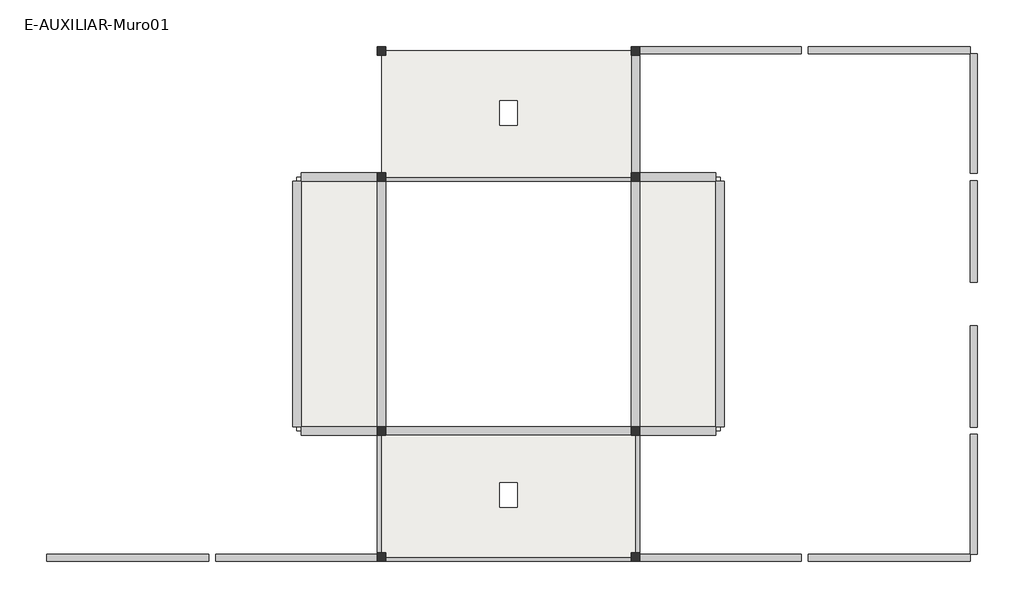
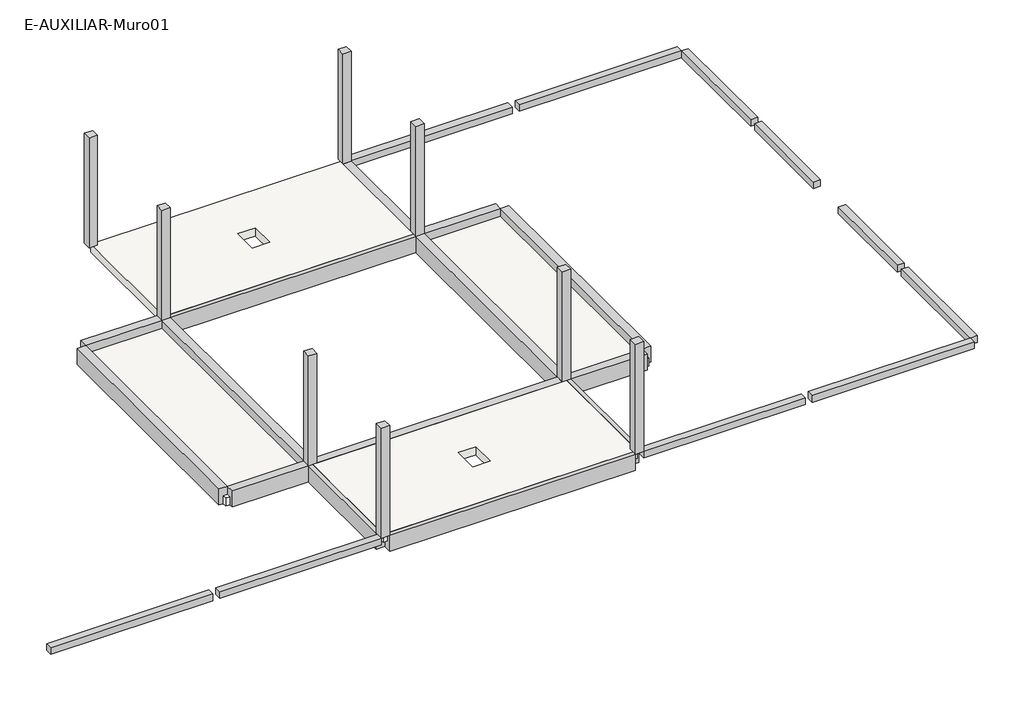
# One storey: 24 beams, 8 columns, 4 slabs.
"""IFC4 building model written with IfcOpenShell, lengths in millimetres."""

from ifc_helpers import new_model, si_unit, frame, origin, place, context, project, spatial, polyline, outline, extrude, faceted_brep, element, save

model = new_model("IFC4")

# Units and contexts
model_context = context("Model", 3, world=origin())
ifc_project = project(units=[si_unit("LENGTHUNIT", "METRE", prefix="MILLI")], contexts=[model_context])

# Site, building, storey
site = spatial("IfcSite", under=ifc_project)
building = spatial("IfcBuilding", under=site)
storey = spatial("IfcBuildingStorey", under=building, Name="E-AUXILIAR-Muro01", Elevation=2730.0)

# Beams
placement = place(None, origin())
element("IfcBeam", 1, ObjectType="E-VIGA-Hormigon : E-VIGA-Hormigon", at=placement, inside=storey, context=model_context, shape_type="Brep", body=[
    faceted_brep([(-24150.0, -13350.0, 2130.0), (-24150.0, -13350.0, 2730.0), (-24150.0, -4650.0, 2730.0), (-24150.0, -4650.0, 2130.0), (-23850.0, -13350.0, 2130.0), (-24000.0, -13350.0, 2130.0), (-24000.0, -4650.0, 2130.0), (-23850.0, -4650.0, 2130.0), (-23850.0, -13350.0, 2730.0), (-23850.0, -13350.0, 2430.0), (-23850.0, -4650.0, 2430.0), (-23850.0, -4650.0, 2730.0)], [[[0, 1, 2, 3]], [[4, 5, 0, 3, 6, 7]], [[8, 9, 4, 7, 10, 11]], [[1, 8, 11, 2]], [[2, 11, 10, 7, 6, 3]], [[1, 0, 5, 4, 9, 8]]]),
])
element("IfcBeam", 2, ObjectType="E-VIGA-Hormigon : E-VIGA-Hormigon", at=placement, inside=storey, context=model_context, shape_type="Brep", body=[
    faceted_brep([(-21150.0, -13350.0, 2130.0), (-21150.0, -13350.0, 2430.0), (-21150.0, -13350.0, 2730.0), (-21150.0, -4650.0, 2730.0), (-21150.0, -4650.0, 2430.0), (-21150.0, -4650.0, 2130.0), (-20850.0, -13350.0, 2130.0), (-21000.0, -13350.0, 2130.0), (-21000.0, -4650.0, 2130.0), (-20850.0, -4650.0, 2130.0), (-20850.0, -13350.0, 2730.0), (-20850.0, -4650.0, 2730.0)], [[[0, 1, 2, 3, 4, 5]], [[6, 7, 0, 5, 8, 9]], [[10, 6, 9, 11]], [[2, 10, 11, 3]], [[3, 11, 9, 8, 5, 4]], [[2, 1, 0, 7, 6, 10]]]),
])
element("IfcBeam", 3, ObjectType="E-VIGA-Hormigon : E-VIGA-Hormigon", at=placement, inside=storey, context=model_context, shape_type="Brep", body=[
    faceted_brep([(-12150.0, -13350.0, 2130.0), (-12150.0, -13350.0, 2730.0), (-12150.0, -4650.0, 2730.0), (-12150.0, -4650.0, 2130.0), (-11850.0, -13350.0, 2130.0), (-12000.0, -13350.0, 2130.0), (-12000.0, -4650.0, 2130.0), (-11850.0, -4650.0, 2130.0), (-11850.0, -13350.0, 2730.0), (-11850.0, -13350.0, 2430.0), (-11850.0, -4650.0, 2430.0), (-11850.0, -4650.0, 2730.0)], [[[0, 1, 2, 3]], [[4, 5, 0, 3, 6, 7]], [[8, 9, 4, 7, 10, 11]], [[1, 8, 11, 2]], [[2, 11, 10, 7, 6, 3]], [[1, 0, 5, 4, 9, 8]]]),
])
element("IfcBeam", 4, ObjectType="E-VIGA-Hormigon : E-VIGA-Hormigon", at=placement, inside=storey, context=model_context, shape_type="Brep", body=[
    faceted_brep([(-9150.0, -13350.0, 2130.0), (-9150.0, -13350.0, 2430.0), (-9150.0, -13350.0, 2730.0), (-9150.0, -4650.0, 2730.0), (-9150.0, -4650.0, 2430.0), (-9150.0, -4650.0, 2130.0), (-8850.0, -13350.0, 2130.0), (-9000.0, -13350.0, 2130.0), (-9000.0, -4650.0, 2130.0), (-8850.0, -4650.0, 2130.0), (-8850.0, -13350.0, 2730.0), (-8850.0, -4650.0, 2730.0)], [[[0, 1, 2, 3, 4, 5]], [[6, 7, 0, 5, 8, 9]], [[10, 6, 9, 11]], [[2, 10, 11, 3]], [[3, 11, 9, 8, 5, 4]], [[2, 1, 0, 7, 6, 10]]]),
])
element("IfcBeam", 5, ObjectType="E-VIGA-Hormigon : E-VIGA-Hormigon", at=placement, inside=storey, context=model_context, shape_type="SweptSolid", body=[
    extrude(outline(polyline([(-4650.0, 2730.0), (-4350.0, 2730.0), (-4350.0, 2130.0), (-4500.0, 2130.0), (-4500.0, 2430.0), (-4650.0, 2430.0), (-4650.0, 2730.0)])), frame((-23850.0, 0.0, 0.0), z_axis=(1.0, 0.0, 0.0), x_axis=(0.0, 1.0, 0.0)), (0.0, 0.0, 1.0), 2700.0),
])
element("IfcBeam", 6, ObjectType="E-VIGA-Hormigon : E-VIGA-Hormigon", at=placement, inside=storey, context=model_context, shape_type="SweptSolid", body=[
    extrude(outline(polyline([(-4350.0, 2130.0), (-4650.0, 2130.0), (-4650.0, 2730.0), (-4500.0, 2730.0), (-4500.0, 2430.0), (-4350.0, 2430.0), (-4350.0, 2130.0)])), frame((-20850.0, 0.0, 0.0), z_axis=(1.0, 0.0, 0.0), x_axis=(0.0, 1.0, 0.0)), (0.0, 0.0, 1.0), 8700.0),
])
element("IfcBeam", 7, ObjectType="E-VIGA-Hormigon : E-VIGA-Hormigon", at=placement, inside=storey, context=model_context, shape_type="SweptSolid", body=[
    extrude(outline(polyline([(-4650.0, 2730.0), (-4350.0, 2730.0), (-4350.0, 2130.0), (-4500.0, 2130.0), (-4500.0, 2430.0), (-4650.0, 2430.0), (-4650.0, 2730.0)])), frame((-11850.0, 0.0, 0.0), z_axis=(1.0, 0.0, 0.0), x_axis=(0.0, 1.0, 0.0)), (0.0, 0.0, 1.0), 2700.0),
])
element("IfcBeam", 8, ObjectType="E-VIGA-Hormigon : E-VIGA-Hormigon", at=placement, inside=storey, context=model_context, shape_type="SweptSolid", body=[
    extrude(outline(polyline([(-13650.0, 2130.0), (-13650.0, 2730.0), (-13350.0, 2730.0), (-13350.0, 2430.0), (-13500.0, 2430.0), (-13500.0, 2130.0), (-13650.0, 2130.0)])), frame((-23850.0, 0.0, 0.0), z_axis=(1.0, 0.0, 0.0), x_axis=(0.0, 1.0, 0.0)), (0.0, 0.0, 1.0), 2700.0),
])
element("IfcBeam", 9, ObjectType="E-VIGA-Hormigon : E-VIGA-Hormigon", at=placement, inside=storey, context=model_context, shape_type="Brep", body=[
    faceted_brep([(-12150.0, -13350.0, 2130.0), (-20850.0, -13350.0, 2130.0), (-20850.0, -13350.0, 2730.0), (-12150.0, -13350.0, 2730.0), (-12150.0, -13650.0, 2130.0), (-20850.0, -13650.0, 2130.0), (-12150.0, -13650.0, 2730.0), (-20850.0, -13650.0, 2730.0), (-20850.0, -13650.0, 2430.0), (-12150.0, -13650.0, 2430.0), (-20850.0, -13500.0, 2730.0), (-12150.0, -13500.0, 2730.0)], [[[0, 1, 2, 3]], [[4, 5, 1, 0]], [[6, 7, 8, 5, 4, 9]], [[3, 2, 10, 7, 6, 11]], [[3, 11, 6, 9, 4, 0]], [[2, 1, 5, 8, 7, 10]]]),
])
element("IfcBeam", 10, ObjectType="E-VIGA-Hormigon : E-VIGA-Hormigon", at=placement, inside=storey, context=model_context, shape_type="SweptSolid", body=[
    extrude(outline(polyline([(-13650.0, 2130.0), (-13650.0, 2730.0), (-13350.0, 2730.0), (-13350.0, 2430.0), (-13500.0, 2430.0), (-13500.0, 2130.0), (-13650.0, 2130.0)])), frame((-11850.0, 0.0, 0.0), z_axis=(1.0, 0.0, 0.0), x_axis=(0.0, 1.0, 0.0)), (0.0, 0.0, 1.0), 2700.0),
])
element("IfcBeam", 11, ObjectType="E-VIGA-Hormigon : E-VIGA-Hormigon", at=placement, inside=storey, context=model_context, shape_type="SweptSolid", body=[
    extrude(outline(polyline([(2730.0, -21150.0), (2130.0, -21150.0), (2130.0, -20850.0), (2430.0, -20850.0), (2430.0, -21000.0), (2730.0, -21000.0), (2730.0, -21150.0)])), frame((0.0, -17825.0, 0.0), z_axis=(0.0, 1.0, 0.0), x_axis=(0.0, 0.0, 1.0)), (0.0, 0.0, 1.0), 4175.0),
])
element("IfcBeam", 12, ObjectType="E-VIGA-Hormigon : E-VIGA-Hormigon", at=placement, inside=storey, context=model_context, shape_type="Brep", body=[
    faceted_brep([(-11850.0, -4350.0, 2130.0), (-11850.0, -175.0, 2130.0), (-11850.0, -175.0, 2730.0), (-11850.0, -4350.0, 2730.0), (-12150.0, -4350.0, 2130.0), (-12150.0, -175.0, 2130.0), (-12150.0, -4350.0, 2730.0), (-12150.0, -175.0, 2730.0), (-12150.0, -175.0, 2430.0), (-12150.0, -4350.0, 2430.0), (-12000.0, -175.0, 2730.0), (-12000.0, -4350.0, 2730.0)], [[[0, 1, 2, 3]], [[4, 5, 1, 0]], [[6, 7, 8, 5, 4, 9]], [[3, 2, 10, 7, 6, 11]], [[3, 11, 6, 9, 4, 0]], [[2, 1, 5, 8, 7, 10]]]),
])
element("IfcBeam", 13, ObjectType="E-VIGA-Hormigon : E-VIGA-Hormigon", at=placement, inside=storey, context=model_context, shape_type="SweptSolid", body=[
    extrude(outline(polyline([(2130.0, -12150.0), (2130.0, -11850.0), (2730.0, -11850.0), (2730.0, -12000.0), (2430.0, -12000.0), (2430.0, -12150.0), (2130.0, -12150.0)])), frame((0.0, -17825.0, 0.0), z_axis=(0.0, 1.0, 0.0), x_axis=(0.0, 0.0, 1.0)), (0.0, 0.0, 1.0), 4175.0),
])
element("IfcBeam", 14, ObjectType="E-VIGA-Hormigon : E-VIGA-Hormigon", at=placement, inside=storey, context=model_context, shape_type="SweptSolid", body=[
    extrude(outline(polyline([(-17825.0, 2130.0), (-18125.0, 2130.0), (-18125.0, 2730.0), (-17975.0, 2730.0), (-17975.0, 2430.0), (-17825.0, 2430.0), (-17825.0, 2130.0)])), frame((-20850.0, 0.0, 0.0), z_axis=(1.0, 0.0, 0.0), x_axis=(0.0, 1.0, 0.0)), (0.0, 0.0, 1.0), 8700.0),
])
element("IfcBeam", 15, ObjectType="E-VIGA-Hormigon : E-VIGA-Hormigon", at=placement, inside=storey, context=model_context, shape_type="SweptSolid", body=[
    extrude(outline(polyline([(-125.0, -13625.0), (125.0, -13625.0), (125.0, -17875.0), (-125.0, -17875.0), (-125.0, -13625.0)])), frame((0.0, 0.0, 2480.0), z_axis=(0.0, 0.0, 1.0), x_axis=(1.0, 0.0, 0.0)), (0.0, 0.0, 1.0), 250.0),
])
element("IfcBeam", 16, ObjectType="E-VIGA-Hormigon : E-VIGA-Hormigon", at=placement, inside=storey, context=model_context, shape_type="SweptSolid", body=[
    extrude(outline(polyline([(125.0, -13375.0), (-125.0, -13375.0), (-125.0, -9775.0), (125.0, -9775.0), (125.0, -13375.0)])), frame((0.0, 0.0, 2480.0), z_axis=(0.0, 0.0, 1.0), x_axis=(1.0, 0.0, 0.0)), (0.0, 0.0, 1.0), 250.0),
])
element("IfcBeam", 17, ObjectType="E-VIGA-Hormigon : E-VIGA-Hormigon", at=placement, inside=storey, context=model_context, shape_type="SweptSolid", body=[
    extrude(outline(polyline([(-125.0, -4625.0), (125.0, -4625.0), (125.0, -8225.0), (-125.0, -8225.0), (-125.0, -4625.0)])), frame((0.0, 0.0, 2480.0), z_axis=(0.0, 0.0, 1.0), x_axis=(1.0, 0.0, 0.0)), (0.0, 0.0, 1.0), 250.0),
])
element("IfcBeam", 18, ObjectType="E-VIGA-Hormigon : E-VIGA-Hormigon", at=placement, inside=storey, context=model_context, shape_type="SweptSolid", body=[
    extrude(outline(polyline([(125.0, -125.0), (125.0, -4375.0), (-125.0, -4375.0), (-125.0, -125.0), (125.0, -125.0)])), frame((0.0, 0.0, 2480.0), z_axis=(0.0, 0.0, 1.0), x_axis=(1.0, 0.0, 0.0)), (0.0, 0.0, 1.0), 250.0),
])
element("IfcBeam", 19, ObjectType="E-VIGA-Hormigon : E-VIGA-Hormigon", at=placement, inside=storey, context=model_context, shape_type="SweptSolid", body=[
    extrude(outline(polyline([(-5875.0, 125.0), (-125.0, 125.0), (-125.0, -125.0), (-5875.0, -125.0), (-5875.0, 125.0)])), frame((0.0, 0.0, 2480.0), z_axis=(0.0, 0.0, 1.0), x_axis=(1.0, 0.0, 0.0)), (0.0, 0.0, 1.0), 250.0),
])
element("IfcBeam", 20, ObjectType="E-VIGA-Hormigon : E-VIGA-Hormigon", at=placement, inside=storey, context=model_context, shape_type="SweptSolid", body=[
    extrude(outline(polyline([(-6125.0, 125.0), (-6125.0, -125.0), (-11850.0, -125.0), (-11850.0, 125.0), (-6125.0, 125.0)])), frame((0.0, 0.0, 2480.0), z_axis=(0.0, 0.0, 1.0), x_axis=(1.0, 0.0, 0.0)), (0.0, 0.0, 1.0), 250.0),
])
element("IfcBeam", 21, ObjectType="E-VIGA-Hormigon : E-VIGA-Hormigon", at=placement, inside=storey, context=model_context, shape_type="SweptSolid", body=[
    extrude(outline(polyline([(-27125.0, -18125.0), (-32875.0, -18125.0), (-32875.0, -17875.0), (-27125.0, -17875.0), (-27125.0, -18125.0)])), frame((0.0, 0.0, 2480.0), z_axis=(0.0, 0.0, 1.0), x_axis=(1.0, 0.0, 0.0)), (0.0, 0.0, 1.0), 250.0),
])
element("IfcBeam", 22, ObjectType="E-VIGA-Hormigon : E-VIGA-Hormigon", at=placement, inside=storey, context=model_context, shape_type="SweptSolid", body=[
    extrude(outline(polyline([(-26875.0, -18125.0), (-26875.0, -17875.0), (-21150.0, -17875.0), (-21150.0, -18125.0), (-26875.0, -18125.0)])), frame((0.0, 0.0, 2480.0), z_axis=(0.0, 0.0, 1.0), x_axis=(1.0, 0.0, 0.0)), (0.0, 0.0, 1.0), 250.0),
])
element("IfcBeam", 23, ObjectType="E-VIGA-Hormigon : E-VIGA-Hormigon", at=placement, inside=storey, context=model_context, shape_type="SweptSolid", body=[
    extrude(outline(polyline([(-5875.0, -18125.0), (-5875.0, -17875.0), (-125.0, -17875.0), (-125.0, -18125.0), (-5875.0, -18125.0)])), frame((0.0, 0.0, 2480.0), z_axis=(0.0, 0.0, 1.0), x_axis=(1.0, 0.0, 0.0)), (0.0, 0.0, 1.0), 250.0),
])
element("IfcBeam", 24, ObjectType="E-VIGA-Hormigon : E-VIGA-Hormigon", at=placement, inside=storey, context=model_context, shape_type="SweptSolid", body=[
    extrude(outline(polyline([(-6125.0, -17875.0), (-6125.0, -18125.0), (-11850.0, -18125.0), (-11850.0, -17875.0), (-6125.0, -17875.0)])), frame((0.0, 0.0, 2480.0), z_axis=(0.0, 0.0, 1.0), x_axis=(1.0, 0.0, 0.0)), (0.0, 0.0, 1.0), 250.0),
])

# Columns
element("IfcColumn", 25, ObjectType="Hormigón-Cuadrado-Pilar : PILAR 30X30", at=placement, inside=storey, context=model_context, shape_type="SweptSolid", body=[
    extrude(outline(polyline([(-20850.0, -4350.0), (-20850.0, -4650.0), (-21150.0, -4650.0), (-21150.0, -4350.0), (-20850.0, -4350.0)])), frame((0.0, 0.0, 2730.0), z_axis=(0.0, 0.0, 1.0), x_axis=(1.0, 0.0, 0.0)), (0.0, 0.0, 1.0), 4120.0),
])
element("IfcColumn", 26, ObjectType="Hormigón-Cuadrado-Pilar : PILAR 30X30", at=placement, inside=storey, context=model_context, shape_type="Brep", body=[
    faceted_brep([(-11850.0, -4350.0, 2730.0), (-11850.0, -4650.0, 2730.0), (-12150.0, -4650.0, 2730.0), (-12150.0, -4350.0, 2730.0), (-12000.0, -4350.0, 2730.0), (-11850.0, -4350.0, 6850.0), (-11850.0, -4650.0, 6850.0), (-12150.0, -4650.0, 6850.0), (-12150.0, -4350.0, 6850.0)], [[[0, 1, 2, 3, 4]], [[5, 6, 1, 0]], [[6, 7, 2, 1]], [[7, 8, 3, 2]], [[8, 5, 0, 4, 3]], [[5, 8, 7, 6]]]),
])
element("IfcColumn", 27, ObjectType="Hormigón-Cuadrado-Pilar : PILAR 30X30", at=placement, inside=storey, context=model_context, shape_type="Brep", body=[
    faceted_brep([(-11850.0, -13350.0, 2730.0), (-11850.0, -13650.0, 2730.0), (-12150.0, -13650.0, 2730.0), (-12150.0, -13500.0, 2730.0), (-12150.0, -13350.0, 2730.0), (-11850.0, -13350.0, 6850.0), (-11850.0, -13650.0, 6850.0), (-12150.0, -13650.0, 6850.0), (-12150.0, -13350.0, 6850.0)], [[[0, 1, 2, 3, 4]], [[5, 6, 1, 0]], [[6, 7, 2, 1]], [[7, 8, 4, 3, 2]], [[8, 5, 0, 4]], [[5, 8, 7, 6]]]),
])
element("IfcColumn", 28, ObjectType="Hormigón-Cuadrado-Pilar : PILAR 30X30", at=placement, inside=storey, context=model_context, shape_type="Brep", body=[
    faceted_brep([(-20850.0, -13350.0, 2730.0), (-20850.0, -13500.0, 2730.0), (-20850.0, -13650.0, 2730.0), (-21150.0, -13650.0, 2730.0), (-21150.0, -13350.0, 2730.0), (-20850.0, -13350.0, 6850.0), (-20850.0, -13650.0, 6850.0), (-21150.0, -13650.0, 6850.0), (-21150.0, -13350.0, 6850.0)], [[[0, 1, 2, 3, 4]], [[5, 6, 2, 1, 0]], [[6, 7, 3, 2]], [[7, 8, 4, 3]], [[8, 5, 0, 4]], [[5, 8, 7, 6]]]),
])
element("IfcColumn", 29, ObjectType="Hormigón-Cuadrado-Pilar : PILAR 30X30", at=placement, inside=storey, context=model_context, shape_type="SweptSolid", body=[
    extrude(outline(polyline([(-20850.0, -17825.0), (-20850.0, -18125.0), (-21150.0, -18125.0), (-21150.0, -17825.0), (-20850.0, -17825.0)])), frame((0.0, 0.0, 2730.0), z_axis=(0.0, 0.0, 1.0), x_axis=(1.0, 0.0, 0.0)), (0.0, 0.0, 1.0), 4120.0),
])
element("IfcColumn", 30, ObjectType="Hormigón-Cuadrado-Pilar : PILAR 30X30", at=placement, inside=storey, context=model_context, shape_type="SweptSolid", body=[
    extrude(outline(polyline([(-12150.0, -17825.0), (-11850.0, -17825.0), (-11850.0, -18125.0), (-12150.0, -18125.0), (-12150.0, -17825.0)])), frame((0.0, 0.0, 2730.0), z_axis=(0.0, 0.0, 1.0), x_axis=(1.0, 0.0, 0.0)), (0.0, 0.0, 1.0), 4120.0),
])
element("IfcColumn", 31, ObjectType="Hormigón-Cuadrado-Pilar : PILAR 30X30", at=placement, inside=storey, context=model_context, shape_type="SweptSolid", body=[
    extrude(outline(polyline([(-20850.0, -175.0), (-21150.0, -175.0), (-21150.0, 125.0), (-20850.0, 125.0), (-20850.0, -175.0)])), frame((0.0, 0.0, 2730.0), z_axis=(0.0, 0.0, 1.0), x_axis=(1.0, 0.0, 0.0)), (0.0, 0.0, 1.0), 4120.0),
])
element("IfcColumn", 32, ObjectType="Hormigón-Cuadrado-Pilar : PILAR 30X30", at=placement, inside=storey, context=model_context, shape_type="Brep", body=[
    faceted_brep([(-12150.0, -175.0, 2730.0), (-12150.0, 125.0, 2730.0), (-11850.0, 125.0, 2730.0), (-11850.0, -175.0, 2730.0), (-12000.0, -175.0, 2730.0), (-12150.0, -175.0, 6850.0), (-12150.0, 125.0, 6850.0), (-11850.0, 125.0, 6850.0), (-11850.0, -175.0, 6850.0)], [[[0, 1, 2, 3, 4]], [[5, 6, 1, 0]], [[6, 7, 2, 1]], [[7, 8, 3, 2]], [[8, 5, 0, 4, 3]], [[5, 8, 7, 6]]]),
])

# Slabs
element("IfcSlab", 33, ObjectType="FORJADO 1_PABLO", at=placement, inside=storey, context=model_context, shape_type="Brep", body=[
    faceted_brep([(-21000.0, -4500.0, 2430.0), (-21000.0, -4350.0, 2430.0), (-21000.0, -175.0, 2430.0), (-21000.0, -25.0, 2430.0), (-20850.0, -25.0, 2430.0), (-12150.0, -25.0, 2430.0), (-12000.0, -25.0, 2430.0), (-12000.0, -175.0, 2430.0), (-12150.0, -175.0, 2430.0), (-12150.0, -4350.0, 2430.0), (-12000.0, -4350.0, 2430.0), (-12000.0, -4500.0, 2430.0), (-12150.0, -4500.0, 2430.0), (-20850.0, -4500.0, 2430.0), (-16811.05, -1791.95, 2430.0), (-16811.05, -2668.05, 2430.0), (-16188.95, -2668.05, 2430.0), (-16188.95, -1791.95, 2430.0), (-21000.0, -25.0, 2730.0), (-21000.0, -175.0, 2730.0), (-21000.0, -4350.0, 2730.0), (-21000.0, -4500.0, 2730.0), (-20850.0, -4500.0, 2730.0), (-12150.0, -4500.0, 2730.0), (-12000.0, -4500.0, 2730.0), (-12000.0, -4350.0, 2730.0), (-12150.0, -4350.0, 2730.0), (-12150.0, -175.0, 2730.0), (-12000.0, -175.0, 2730.0), (-12000.0, -25.0, 2730.0), (-12150.0, -25.0, 2730.0), (-20850.0, -25.0, 2730.0), (-16811.05, -2668.05, 2730.0), (-16811.05, -1791.95, 2730.0), (-16188.95, -1791.95, 2730.0), (-16188.95, -2668.05, 2730.0)], [[[0, 1, 2, 3, 4, 5, 6, 7, 8, 9, 10, 11, 12, 13], [14, 15, 16, 17]], [[18, 19, 20, 21, 22, 23, 24, 25, 26, 27, 28, 29, 30, 31], [32, 33, 34, 35]], [[3, 2, 1, 0, 21, 20, 19, 18]], [[6, 5, 4, 3, 18, 31, 30, 29]], [[24, 11, 10, 25]], [[6, 29, 28, 7]], [[0, 13, 12, 11, 24, 23, 22, 21]], [[15, 14, 33, 32]], [[16, 15, 32, 35]], [[17, 16, 35, 34]], [[14, 17, 34, 33]], [[26, 9, 8, 27]], [[9, 26, 25, 10]], [[27, 8, 7, 28]]]),
])
element("IfcSlab", 34, ObjectType="FORJADO 1_PABLO", at=placement, inside=storey, context=model_context, shape_type="Brep", body=[
    faceted_brep([(-12000.0, -13500.0, 2430.0), (-12000.0, -13650.0, 2430.0), (-12000.0, -17825.0, 2430.0), (-12000.0, -17975.0, 2430.0), (-12150.0, -17975.0, 2430.0), (-20850.0, -17975.0, 2430.0), (-21000.0, -17975.0, 2430.0), (-21000.0, -17825.0, 2430.0), (-21000.0, -13650.0, 2430.0), (-21000.0, -13500.0, 2430.0), (-20850.0, -13500.0, 2430.0), (-20850.0, -13650.0, 2430.0), (-12150.0, -13650.0, 2430.0), (-12150.0, -13500.0, 2430.0), (-16188.95, -15331.95, 2430.0), (-16811.05, -15331.95, 2430.0), (-16811.05, -16208.05, 2430.0), (-16188.95, -16208.05, 2430.0), (-12000.0, -17975.0, 2730.0), (-12000.0, -17825.0, 2730.0), (-12000.0, -13650.0, 2730.0), (-12000.0, -13500.0, 2730.0), (-12150.0, -13500.0, 2730.0), (-12150.0, -13650.0, 2730.0), (-20850.0, -13650.0, 2730.0), (-20850.0, -13500.0, 2730.0), (-21000.0, -13500.0, 2730.0), (-21000.0, -13650.0, 2730.0), (-21000.0, -17825.0, 2730.0), (-21000.0, -17975.0, 2730.0), (-20850.0, -17975.0, 2730.0), (-12150.0, -17975.0, 2730.0), (-16811.05, -15331.95, 2730.0), (-16188.95, -15331.95, 2730.0), (-16188.95, -16208.05, 2730.0), (-16811.05, -16208.05, 2730.0)], [[[0, 1, 2, 3, 4, 5, 6, 7, 8, 9, 10, 11, 12, 13], [14, 15, 16, 17]], [[18, 19, 20, 21, 22, 23, 24, 25, 26, 27, 28, 29, 30, 31], [32, 33, 34, 35]], [[3, 2, 1, 0, 21, 20, 19, 18]], [[6, 5, 4, 3, 18, 31, 30, 29]], [[9, 8, 7, 6, 29, 28, 27, 26]], [[21, 0, 13, 22]], [[9, 26, 25, 10]], [[15, 14, 33, 32]], [[16, 15, 32, 35]], [[17, 16, 35, 34]], [[14, 17, 34, 33]], [[23, 12, 11, 24]], [[12, 23, 22, 13]], [[24, 11, 10, 25]]]),
])
element("IfcSlab", 35, ObjectType="FORJADO 1_PABLO", at=placement, inside=storey, context=model_context, shape_type="Brep", body=[
    faceted_brep([(-9000.0, -13500.0, 2130.0), (-9150.0, -13500.0, 2130.0), (-11850.0, -13500.0, 2130.0), (-12000.0, -13500.0, 2130.0), (-12000.0, -13350.0, 2130.0), (-11850.0, -13350.0, 2130.0), (-11850.0, -4650.0, 2130.0), (-12000.0, -4650.0, 2130.0), (-12000.0, -4500.0, 2130.0), (-11850.0, -4500.0, 2130.0), (-9150.0, -4500.0, 2130.0), (-9000.0, -4500.0, 2130.0), (-9000.0, -4650.0, 2130.0), (-9150.0, -4650.0, 2130.0), (-9150.0, -13350.0, 2130.0), (-9000.0, -13350.0, 2130.0), (-12000.0, -13500.0, 2430.0), (-11850.0, -13500.0, 2430.0), (-9150.0, -13500.0, 2430.0), (-9000.0, -13500.0, 2430.0), (-9000.0, -13350.0, 2430.0), (-9150.0, -13350.0, 2430.0), (-9150.0, -4650.0, 2430.0), (-9000.0, -4650.0, 2430.0), (-9000.0, -4500.0, 2430.0), (-9150.0, -4500.0, 2430.0), (-11850.0, -4500.0, 2430.0), (-12000.0, -4500.0, 2430.0), (-12000.0, -4650.0, 2430.0), (-11850.0, -4650.0, 2430.0), (-11850.0, -13350.0, 2430.0), (-12000.0, -13350.0, 2430.0)], [[[0, 1, 2, 3, 4, 5, 6, 7, 8, 9, 10, 11, 12, 13, 14, 15]], [[16, 17, 18, 19, 20, 21, 22, 23, 24, 25, 26, 27, 28, 29, 30, 31]], [[11, 24, 23, 12]], [[19, 0, 15, 20]], [[3, 2, 1, 0, 19, 18, 17, 16]], [[27, 8, 7, 28]], [[3, 16, 31, 4]], [[11, 10, 9, 8, 27, 26, 25, 24]], [[29, 6, 5, 30]], [[6, 29, 28, 7]], [[30, 5, 4, 31]], [[13, 22, 21, 14]], [[22, 13, 12, 23]], [[14, 21, 20, 15]]]),
])
element("IfcSlab", 36, ObjectType="FORJADO 1_PABLO", at=placement, inside=storey, context=model_context, shape_type="Brep", body=[
    faceted_brep([(-21000.0, -13500.0, 2130.0), (-21150.0, -13500.0, 2130.0), (-23850.0, -13500.0, 2130.0), (-24000.0, -13500.0, 2130.0), (-24000.0, -13350.0, 2130.0), (-23850.0, -13350.0, 2130.0), (-23850.0, -4650.0, 2130.0), (-24000.0, -4650.0, 2130.0), (-24000.0, -4500.0, 2130.0), (-23850.0, -4500.0, 2130.0), (-21150.0, -4500.0, 2130.0), (-21000.0, -4500.0, 2130.0), (-21000.0, -4650.0, 2130.0), (-21150.0, -4650.0, 2130.0), (-21150.0, -13350.0, 2130.0), (-21000.0, -13350.0, 2130.0), (-24000.0, -13500.0, 2430.0), (-23850.0, -13500.0, 2430.0), (-21150.0, -13500.0, 2430.0), (-21000.0, -13500.0, 2430.0), (-21000.0, -13350.0, 2430.0), (-21150.0, -13350.0, 2430.0), (-21150.0, -4650.0, 2430.0), (-21000.0, -4650.0, 2430.0), (-21000.0, -4500.0, 2430.0), (-21150.0, -4500.0, 2430.0), (-23850.0, -4500.0, 2430.0), (-24000.0, -4500.0, 2430.0), (-24000.0, -4650.0, 2430.0), (-23850.0, -4650.0, 2430.0), (-23850.0, -13350.0, 2430.0), (-24000.0, -13350.0, 2430.0)], [[[0, 1, 2, 3, 4, 5, 6, 7, 8, 9, 10, 11, 12, 13, 14, 15]], [[16, 17, 18, 19, 20, 21, 22, 23, 24, 25, 26, 27, 28, 29, 30, 31]], [[11, 24, 23, 12]], [[19, 0, 15, 20]], [[3, 2, 1, 0, 19, 18, 17, 16]], [[27, 8, 7, 28]], [[3, 16, 31, 4]], [[11, 10, 9, 8, 27, 26, 25, 24]], [[29, 6, 5, 30]], [[6, 29, 28, 7]], [[30, 5, 4, 31]], [[13, 22, 21, 14]], [[22, 13, 12, 23]], [[14, 21, 20, 15]]]),
])

save(model, "model.ifc")

# Revit data of these elements
# Type "E-VIGA-Hormigon : E-VIGA-Hormigon"
#   Numeration [instance default] = ""
#   Length [instance default] = 3.000 m
#   AnchoViga [instance default] = 0.200 m
#   AltoViga [instance default] = 0.300 m
# Type "Hormigón-Cuadrado-Pilar : PILAR 30X30"
#   b = 0.300 m
#   Structural Material [instance default] = Hormigón - Hormigón moldeado in situ
# Type "FORJADO 1_PABLO"
#   Function = 0
#   Layers, outside or top first: 0.140 m "Hormigón, moldeado in situ" (function 1); 0.160 m "Forjado vigueta semirresistente y bovedilla cerámica" (function 1)
# Elements 1, 2, 3, 4, 5, 6, 7, 8, 9, 10, 11, 12, 13, 14 (IfcBeam, "E-VIGA-Hormigon : E-VIGA-Hormigon")
#   Comments = ""
#   Numeration = ""
#   AnchoViga = 0.300 m
#   AltoViga = 0.600 m
#   Phase Created = Nueva construcción
#   Materials on its faces: "Concrete, Cast-in-Place, Gray"
# Elements 15, 16, 17, 18, 19, 20, 21, 22, 23, 24 (IfcBeam, "E-VIGA-Hormigon : E-VIGA-Hormigon")
#   Comments = ""
#   Numeration = ""
#   AnchoViga = 0.250 m
#   AltoViga = 0.250 m
#   Phase Created = Nueva construcción
#   Materials on its faces: "Concrete, Cast-in-Place, Gray"
# Elements 25, 26, 27, 28, 29, 30, 31, 32 (IfcColumn, "Hormigón-Cuadrado-Pilar : PILAR 30X30")
#   Comments = ""
#   Structural Material = Hormigón - Hormigón moldeado in situ
#   Phase Created = Nueva construcción
#   Materials on its faces: "Hormigón - Hormigón moldeado in situ"
# Element 33 (IfcSlab, "FORJADO 1_PABLO")
#   built-in parameter 1001955 = -1.5708 (stored number, unit not read)
#   Height Offset From Level = 0.000 m
#   built-in parameter 1001954 = 1
#   Phase Created = Nueva construcción
#   Materials on its faces: "Forjado vigueta semirresistente y bovedilla cerámica", "Hormigón, moldeado in situ"
# Element 34 (IfcSlab, "FORJADO 1_PABLO")
#   Height Offset From Level = 0.000 m
#   built-in parameter 1001954 = 1
#   Phase Created = Nueva construcción
#   Materials on its faces: "Forjado vigueta semirresistente y bovedilla cerámica", "Hormigón, moldeado in situ"
# Element 35 (IfcSlab, "FORJADO 1_PABLO")
#   Height Offset From Level = -0.300 m
#   built-in parameter 1001954 = 1
#   Phase Created = Nueva construcción
#   Materials on its faces: "Forjado vigueta semirresistente y bovedilla cerámica", "Hormigón, moldeado in situ"
# Element 36 (IfcSlab, "FORJADO 1_PABLO")
#   Comments = ""
#   Height Offset From Level = -0.300 m
#   built-in parameter 1001954 = 1
#   Phase Created = Nueva construcción
#   Materials on its faces: "Forjado vigueta semirresistente y bovedilla cerámica", "Hormigón, moldeado in situ"
# Materials
#   "Hormigón - Hormigón moldeado in situ": class "Hormigón", colour RGB 192 192 192, transparency 0, Cost = 0
#   "Hormigón, moldeado in situ": class "Hormigón", colour RGB 192 192 192, transparency 0, Description = "material físico", Cost = 0
#   "Forjado vigueta semirresistente y bovedilla cerámica": class "Albañilería", colour RGB 120 120 120, transparency 0, Description = "Ladrillo hueco", Cost = 0
#   "Concrete, Cast-in-Place, Gray": class "Concrete", colour RGB 129 132 118, transparency 0, Description = "Cast-in-place concrete", Cost = 0
